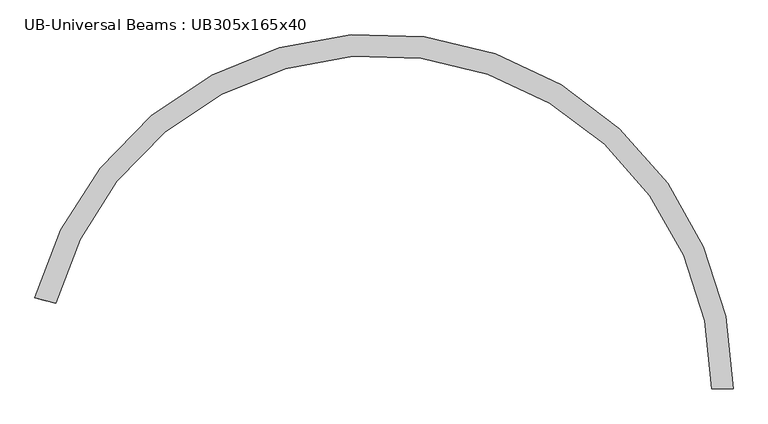
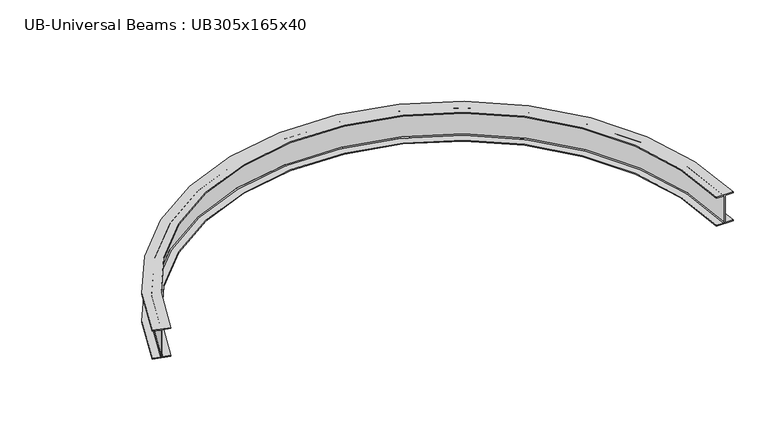
"""IFC4 building model written with IfcOpenShell, lengths in millimetres: beam geometry, UB-Universal Beams : UB305x165x40."""

import ifcopenshell
import ifcopenshell.guid

model = None  # the IFC model being written
_history = None  # IfcOwnerHistory: only IFC2X3 demands one
_inside = {}  # id of a spatial element -> (the spatial element, [elements in it])
_under = {}  # id of a project, library or spatial element -> (it, [spatial elements below it])
_declared = {}  # id of a project -> (the project, [libraries it declares])
_typed = {}  # id of a type object -> (the type object, [elements of that type])
_made_of = {}  # id of a material, layer set ... -> (it, [elements and type objects made of it])


def new_model(schema):
    """Start an empty IFC model of exactly this schema.

    Asked for "IFC4X3", IfcOpenShell would pick the latest addendum, in which some entities
    have other attributes; the version numbers below select the first issue.
    IFC2X3 requires an IfcOwnerHistory on every rooted entity: one is made here for all.
    """
    global model, _history
    if schema == "IFC4X3":
        model = ifcopenshell.file(schema_version=(4, 3, 0, 0))
    else:
        model = ifcopenshell.file(schema=schema)
    _inside.clear()
    _under.clear()
    _declared.clear()
    _typed.clear()
    _made_of.clear()
    _history = None
    if model.schema == "IFC2X3":
        org = make("IfcOrganization", Name="unknown")
        user = make(
            "IfcPersonAndOrganization",
            ThePerson=make("IfcPerson", FamilyName="unknown"),
            TheOrganization=org,
        )
        app = make(
            "IfcApplication",
            ApplicationDeveloper=org,
            Version="unknown",
            ApplicationFullName="unknown",
            ApplicationIdentifier="unknown",
        )
        _history = make(
            "IfcOwnerHistory",
            OwningUser=user,
            OwningApplication=app,
            ChangeAction="ADDED",
            CreationDate=0,
        )
    return model


def make(cls, **values):
    """One entity of the class cls with the attributes given. An attribute that is None is left unset."""
    return model.create_entity(
        cls, **{name: value for name, value in values.items() if value is not None}
    )


def rooted(cls, **values):
    """An entity with a GlobalId (a new one), such as an element, a storey or a relation."""
    return make(cls, GlobalId=ifcopenshell.guid.new(), OwnerHistory=_history, **values)


def si_unit(unit_type, name, prefix=None):
    """IfcSIUnit, for example si_unit("LENGTHUNIT", "METRE", prefix="MILLI")."""
    return make("IfcSIUnit", UnitType=unit_type, Prefix=prefix, Name=name)


def assignment(units):
    """IfcUnitAssignment: the units of a project."""
    return None if units is None else make("IfcUnitAssignment", Units=units)


def point(xyz):
    """IfcCartesianPoint."""
    return None if xyz is None else make("IfcCartesianPoint", Coordinates=xyz)


def direction(xyz):
    """IfcDirection."""
    return None if xyz is None else make("IfcDirection", DirectionRatios=xyz)


def frame(location, z_axis=None, x_axis=None):
    """IfcAxis2Placement3D, a coordinate frame: its origin and axes. An axis left out is left unset."""
    return make(
        "IfcAxis2Placement3D",
        Location=point(location),
        Axis=direction(z_axis),
        RefDirection=direction(x_axis),
    )


def origin():
    """The frame at (0, 0, 0) with its axes left unset."""
    return frame((0.0, 0.0, 0.0))


def place(relative_to, where):
    """IfcLocalPlacement: puts the frame where relative to a parent placement (None: the world)."""
    return make(
        "IfcLocalPlacement", PlacementRelTo=relative_to, RelativePlacement=where
    )


def context(
    kind, dimensions, precision=None, world=None, true_north=None, identifier=None
):
    """IfcGeometricRepresentationContext, for example the 3D "Model" context."""
    return make(
        "IfcGeometricRepresentationContext",
        ContextIdentifier=identifier,
        ContextType=kind,
        CoordinateSpaceDimension=dimensions,
        Precision=precision,
        WorldCoordinateSystem=world,
        TrueNorth=true_north,
    )


def project(units=None, contexts=None):
    """IfcProject with its units and contexts."""
    return rooted(
        "IfcProject",
        Name="project",
        RepresentationContexts=contexts,
        UnitsInContext=assignment(units),
    )


def spatial(cls, under=None, at=None, **own):
    """A site, building, storey or space (cls), placed at a placement, below another one or the project."""
    s = rooted(cls, ObjectPlacement=at, **own)
    if under is not None:
        _under.setdefault(under.id(), (under, []))[1].append(s)
    return s


def polyline(points):
    """IfcPolyline through the points."""
    return make("IfcPolyline", Points=[point(p) for p in points])


def circle_curve(where, radius):
    """IfcCircle in the frame where."""
    return make("IfcCircle", Position=where, Radius=radius)


def ellipse_curve(where, semi_axis1, semi_axis2):
    """IfcEllipse in the frame where."""
    return make(
        "IfcEllipse", Position=where, SemiAxis1=semi_axis1, SemiAxis2=semi_axis2
    )


def trimmed(basis, trim1, trim2, sense, master):
    """IfcTrimmedCurve: the piece of a basis curve between two trims."""
    return make(
        "IfcTrimmedCurve",
        BasisCurve=basis,
        Trim1=trim1,
        Trim2=trim2,
        SenseAgreement=sense,
        MasterRepresentation=master,
    )


def shape(context_of_items, identifier, shape_type, items):
    """IfcShapeRepresentation: the items that make up one representation, for example the "Body"."""
    return make(
        "IfcShapeRepresentation",
        ContextOfItems=context_of_items,
        RepresentationIdentifier=identifier,
        RepresentationType=shape_type,
        Items=items,
    )


def source(mapping_origin, context_of_items, identifier, shape_type, items):
    """IfcRepresentationMap: a shape defined once, which mapped items show again and again."""
    return make(
        "IfcRepresentationMap",
        MappingOrigin=mapping_origin,
        MappedRepresentation=shape(context_of_items, identifier, shape_type, items),
    )


def transform(
    local_origin,
    x_axis=None,
    y_axis=None,
    z_axis=None,
    scale=None,
    scale2=None,
    scale3=None,
    uniform=True,
):
    """IfcCartesianTransformationOperator3D, or its non-uniform kind. x_axis, y_axis, z_axis: its Axis1, 2, 3."""
    if uniform:
        return make(
            "IfcCartesianTransformationOperator3D",
            Axis1=direction(x_axis),
            Axis2=direction(y_axis),
            LocalOrigin=point(local_origin),
            Scale=scale,
            Axis3=direction(z_axis),
        )
    return make(
        "IfcCartesianTransformationOperator3DnonUniform",
        Axis1=direction(x_axis),
        Axis2=direction(y_axis),
        LocalOrigin=point(local_origin),
        Scale=scale,
        Axis3=direction(z_axis),
        Scale2=scale2,
        Scale3=scale3,
    )


def mapped(mapping_source, mapping_target):
    """IfcMappedItem: shows the shape of a source again, moved by a transform."""
    return make(
        "IfcMappedItem", MappingSource=mapping_source, MappingTarget=mapping_target
    )


def made_of(thing, what):
    """Note that an element or type object is made of a material, layer set ...; save() writes the relation."""
    if what is not None:
        _made_of.setdefault(what.id(), (what, []))[1].append(thing)
    return thing


def element(
    cls,
    number,
    at=None,
    inside=None,
    cuts=None,
    type_object=None,
    material=None,
    context=None,
    identifier="Body",
    shape_type=None,
    held_by="IfcProductDefinitionShape",
    body=None,
    shapes=None,
    **own,
):
    """One element of the class cls, such as IfcWall. Its Tag is "e" and its number.

    at: its placement. inside: the storey or other place that contains it. cuts: it is an
    opening in that element (IfcRelVoidsElement). A single representation is given by context,
    identifier, shape_type and body (its items); several are given by shapes. held_by: the class
    of the entity that holds the representations. save() writes the other relations.
    """
    e = rooted(cls, Tag="e%d" % number, ObjectPlacement=at, **own)
    if body is not None:
        shapes = [shape(context, identifier, shape_type, body)]
    if shapes is not None:
        e.Representation = make(held_by, Representations=shapes)
    if inside is not None:
        _inside.setdefault(inside.id(), (inside, []))[1].append(e)
    if cuts is not None:
        rooted(
            "IfcRelVoidsElement", RelatingBuildingElement=cuts, RelatedOpeningElement=e
        )
    if type_object is not None:
        _typed.setdefault(type_object.id(), (type_object, []))[1].append(e)
    return made_of(e, material)


def aggregate(whole, parts):
    """IfcRelAggregates: a whole, such as a stair, and the parts it consists of."""
    return rooted("IfcRelAggregates", RelatingObject=whole, RelatedObjects=parts)


def save(model, path):
    """Write the relations noted so far, then the file.

    IfcRelAggregates (storeys below a building ...), IfcRelContainedInSpatialStructure (elements
    in a storey), IfcRelDefinesByType, IfcRelAssociatesMaterial and IfcRelDeclares: one each for
    every whole, place, type object, material and project.
    """
    for whole, parts in _under.values():
        aggregate(whole, parts)
    for where, things in _inside.values():
        rooted(
            "IfcRelContainedInSpatialStructure",
            RelatedElements=things,
            RelatingStructure=where,
        )
    for kind, things in _typed.values():
        rooted("IfcRelDefinesByType", RelatedObjects=things, RelatingType=kind)
    for what, things in _made_of.values():
        rooted("IfcRelAssociatesMaterial", RelatedObjects=things, RelatingMaterial=what)
    for by, libraries in _declared.values():
        rooted("IfcRelDeclares", RelatingContext=by, RelatedDefinitions=libraries)
    model.write(path)


def plane_surface(at):
    """IfcPlane: the flat surface through the origin of the frame at, square to its z axis."""
    return make("IfcPlane", Position=at)


def cylinder_surface(at, radius):
    """IfcCylindricalSurface: all points at the distance radius from the z axis of the frame at."""
    return make("IfcCylindricalSurface", Position=at, Radius=radius)


def revolved_surface(curve, axis_point, axis_direction):
    """IfcSurfaceOfRevolution: the curve turned about the line through axis_point along axis_direction."""
    return make(
        "IfcSurfaceOfRevolution",
        SweptCurve=make("IfcArbitraryOpenProfileDef", ProfileType="CURVE", Curve=curve),
        AxisPosition=make("IfcAxis1Placement", Location=point(axis_point), Axis=direction(axis_direction)),
    )


def advanced_brep(points, edges, surfaces, faces):
    """IfcAdvancedBrep: a solid bounded by faces that lie on surfaces and meet in shared edges.

    An edge is (start, end): straight between two places in points (the first is 0);
    or (start, end, curve); or (start, end, curve, False) where it runs against its curve.
    A face is (place in surfaces, loops), or (place, loops, False) where it looks against
    its surface's normal. A loop lists edges by number (the first is 1), with a minus sign
    where the edge is run from its end to its start. The first loop is the outer one.
    """
    corners = [point(p) for p in points]
    vertices = [make("IfcVertexPoint", VertexGeometry=c) for c in corners]
    made = []
    for start, end, *more in edges:
        made.append(
            make(
                "IfcEdgeCurve",
                EdgeStart=vertices[start],
                EdgeEnd=vertices[end],
                EdgeGeometry=more[0] if more else make("IfcPolyline", Points=[corners[start], corners[end]]),
                SameSense=more[1] if len(more) > 1 else True,
            )
        )
    hull = []
    for where, loops, *sense in faces:
        bounds = []
        for j, loop in enumerate(loops):
            ring = [make("IfcOrientedEdge", EdgeElement=made[abs(k) - 1], Orientation=k > 0) for k in loop]
            bounds.append(
                make(
                    "IfcFaceOuterBound" if j == 0 else "IfcFaceBound",
                    Bound=make("IfcEdgeLoop", EdgeList=ring),
                    Orientation=True,
                )
            )
        hull.append(make("IfcAdvancedFace", Bounds=bounds, FaceSurface=surfaces[where], SameSense=sense[0] if sense else True))
    return make("IfcAdvancedBrep", Outer=make("IfcClosedShell", CfsFaces=hull))


def ub_universal_beams_ub305x165x40_4e4f8f72(model_context):
    return source(origin(), model_context, "Body", "AdvancedBrep", [
        advanced_brep(
        [(2724.4689627, -2641.9689627, -141.5), (2653.8689627, -2641.9689627, -141.5), (2644.9689627, -2641.9689627, -132.6), (2644.9689627, -2641.9689627, 132.6), (2653.8689627, -2641.9689627, 141.5), (2724.4689627, -2641.9689627, 141.5), (2724.4689627, -2641.9689627, 151.7), (2559.4689627, -2641.9689627, 151.7), (2559.4689627, -2641.9689627, 141.5), (2630.0689627, -2641.9689627, 141.5), (2638.9689627, -2641.9689627, 132.6), (2638.9689627, -2641.9689627, -132.6), (2630.0689627, -2641.9689627, -141.5), (2559.4689627, -2641.9689627, -141.5), (2559.4689627, -2641.9689627, -151.7), (2724.4689627, -2641.9689627, -151.7), (-2633.0924312, -1942.2866222, -141.5), (-2633.0924312, -1942.2866222, -151.7), (-2473.6264005, -1984.6609666, -151.7), (-2473.6264005, -1984.6609666, -141.5), (-2541.8585324, -1966.5298835, -141.5), (-2550.4600335, -1964.244237, -132.6), (-2550.4600335, -1964.244237, 132.6), (-2541.8585324, -1966.5298835, 141.5), (-2473.6264005, -1984.6609666, 141.5), (-2473.6264005, -1984.6609666, 151.7), (-2633.0924312, -1942.2866222, 151.7), (-2633.0924312, -1942.2866222, 141.5), (-2564.8602993, -1960.4177053, 141.5), (-2556.2587982, -1962.7033518, 132.6), (-2556.2587982, -1962.7033518, -132.6), (-2564.8602993, -1960.4177053, -141.5)],
        [
            (0, 1),
            (1, 2, circle_curve(frame((2653.8689627, -2641.9689627, -132.6), z_axis=(0.0, 1.0, 0.0), x_axis=(-1.0, 0.0, 0.0)), 8.9)),
            (2, 3),
            (3, 4, circle_curve(frame((2653.8689627, -2641.9689627, 132.6), z_axis=(0.0, 1.0, 0.0), x_axis=(-1.0, 0.0, 0.0)), 8.9)),
            (4, 5),
            (5, 6),
            (6, 7),
            (7, 8),
            (8, 9),
            (9, 10, circle_curve(frame((2630.0689627, -2641.9689627, 132.6), z_axis=(0.0, 1.0, 0.0), x_axis=(-1.0, 0.0, 0.0)), 8.9)),
            (10, 11),
            (11, 12, circle_curve(frame((2630.0689627, -2641.9689627, -132.6), z_axis=(0.0, 1.0, 0.0), x_axis=(-1.0, 0.0, 0.0)), 8.9)),
            (12, 13),
            (13, 14),
            (14, 15),
            (15, 0),
            (16, 17),
            (17, 18),
            (18, 19),
            (19, 20),
            (20, 21, circle_curve(frame((-2541.8585324, -1966.5298835, -132.6), z_axis=(0.2568142086103926, 0.9664607918875021, 0.0), x_axis=(0.9664607918875021, -0.2568142086103926, 0.0)), 8.9)),
            (21, 22),
            (22, 23, circle_curve(frame((-2541.8585324, -1966.5298835, 132.6), z_axis=(0.2568142086103926, 0.9664607918875021, 0.0), x_axis=(0.9664607918875021, -0.2568142086103926, 0.0)), 8.9)),
            (23, 24),
            (24, 25),
            (25, 26),
            (26, 27),
            (27, 28),
            (28, 29, circle_curve(frame((-2564.8602993, -1960.4177053, 132.6), z_axis=(0.2568142086103926, 0.9664607918875021, 0.0), x_axis=(0.9664607918875021, -0.2568142086103926, 0.0)), 8.9)),
            (29, 30),
            (30, 31, circle_curve(frame((-2564.8602993, -1960.4177053, -132.6), z_axis=(0.2568142086103926, 0.9664607918875021, 0.0), x_axis=(0.9664607918875021, -0.2568142086103926, 0.0)), 8.9)),
            (31, 16),
            (0, 16, circle_curve(frame((0.0, -2641.9689627, -141.5), z_axis=(0.0, 0.0, 1.0), x_axis=(0.0, 1.0, 0.0)), 2724.4689627)),
            (31, 1, circle_curve(frame((0.0, -2641.9689627, -141.5), z_axis=(0.0, 0.0, -1.0), x_axis=(0.0, 1.0, 0.0)), 2653.8689627)),
            (30, 2, circle_curve(frame((0.0, -2641.9689627, -132.6), z_axis=(0.0, 0.0, -1.0), x_axis=(0.0, 1.0, 0.0)), 2644.9689627)),
            (29, 3, circle_curve(frame((0.0, -2641.9689627, 132.6), z_axis=(0.0, 0.0, -1.0), x_axis=(0.0, 1.0, 0.0)), 2644.9689627)),
            (28, 4, circle_curve(frame((0.0, -2641.9689627, 141.5), z_axis=(0.0, 0.0, -1.0), x_axis=(0.0, 1.0, 0.0)), 2653.8689627)),
            (27, 5, circle_curve(frame((0.0, -2641.9689627, 141.5), z_axis=(0.0, 0.0, -1.0), x_axis=(0.0, 1.0, 0.0)), 2724.4689627)),
            (26, 6, circle_curve(frame((0.0, -2641.9689627, 151.7), z_axis=(0.0, 0.0, -1.0), x_axis=(0.0, 1.0, 0.0)), 2724.4689627)),
            (25, 7, circle_curve(frame((0.0, -2641.9689627, 151.7), z_axis=(0.0, 0.0, -1.0), x_axis=(0.0, 1.0, 0.0)), 2559.4689627)),
            (24, 8, circle_curve(frame((0.0, -2641.9689627, 141.5), z_axis=(0.0, 0.0, -1.0), x_axis=(0.0, 1.0, 0.0)), 2559.4689627)),
            (23, 9, circle_curve(frame((0.0, -2641.9689627, 141.5), z_axis=(0.0, 0.0, -1.0), x_axis=(0.0, 1.0, 0.0)), 2630.0689627)),
            (22, 10, circle_curve(frame((0.0, -2641.9689627, 132.6), z_axis=(0.0, 0.0, -1.0), x_axis=(0.0, 1.0, 0.0)), 2638.9689627)),
            (21, 11, circle_curve(frame((0.0, -2641.9689627, -132.6), z_axis=(0.0, 0.0, -1.0), x_axis=(0.0, 1.0, 0.0)), 2638.9689627)),
            (20, 12, circle_curve(frame((0.0, -2641.9689627, -141.5), z_axis=(0.0, 0.0, -1.0), x_axis=(0.0, 1.0, 0.0)), 2630.0689627)),
            (19, 13, circle_curve(frame((0.0, -2641.9689627, -141.5), z_axis=(0.0, 0.0, -1.0), x_axis=(0.0, 1.0, 0.0)), 2559.4689627)),
            (18, 14, circle_curve(frame((0.0, -2641.9689627, -151.7), z_axis=(0.0, 0.0, -1.0), x_axis=(0.0, 1.0, 0.0)), 2559.4689627)),
            (17, 15, circle_curve(frame((0.0, -2641.9689627, -151.7), z_axis=(0.0, 0.0, -1.0), x_axis=(0.0, 1.0, 0.0)), 2724.4689627)),
        ],
        [
            plane_surface(frame((2641.9689627, -2641.9689627, 0.0), z_axis=(0.0, -1.0, 0.0), x_axis=(0.0, 0.0, 1.0))),
            plane_surface(frame((-2553.3594159, -1963.4737944, 0.0), z_axis=(-0.25681420861039306, -0.9664607918875021, 0.0), x_axis=(0.0, 0.0, 1.0))),
            plane_surface(frame((0.0, -2641.9689627, -141.5), z_axis=(0.0, 0.0, 1.0), x_axis=(0.0, 1.0, 0.0))),
            revolved_surface(trimmed(ellipse_curve(frame((0.0, 11.9, -132.6), z_axis=(1.0, 0.0, 0.0), x_axis=(0.0, -1.0, 0.0)), 8.9, 8.9), [point((0.0, 3.0, -132.6))], [point((0.0, 11.9, -141.5))], True, "CARTESIAN"), (0.0, -2641.9689627, 0.0), (0.0, 0.0, -1.0)),
            cylinder_surface(frame((0.0, -2641.9689627, 0.0), z_axis=(0.0, 0.0, -1.0), x_axis=(0.0, 1.0, 0.0)), 2644.9689627),
            revolved_surface(trimmed(ellipse_curve(frame((0.0, 11.9, 132.6), z_axis=(1.0, 0.0, 0.0), x_axis=(0.0, -1.0, 0.0)), 8.9, 8.9), [point((0.0, 11.9, 141.5))], [point((0.0, 3.0, 132.6))], True, "CARTESIAN"), (0.0, -2641.9689627, 0.0), (0.0, 0.0, -1.0)),
            plane_surface(frame((0.0, -2641.9689627, 141.5), z_axis=(0.0, 0.0, -1.0), x_axis=(0.0, 1.0, 0.0))),
            cylinder_surface(frame((0.0, -2641.9689627, 0.0), z_axis=(0.0, 0.0, -1.0), x_axis=(0.0, 1.0, 0.0)), 2724.4689627),
            plane_surface(frame((0.0, -2641.9689627, 151.7), z_axis=(0.0, 0.0, 1.0), x_axis=(0.0, 1.0, 0.0))),
            revolved_surface(polyline([(0.0, -82.5, 141.5), (0.0, -82.5, 151.7)]), (0.0, -2641.9689627, 0.0), (0.0, 0.0, -1.0)),
            revolved_surface(trimmed(ellipse_curve(frame((0.0, -11.9, 132.6), z_axis=(1.0, 0.0, 0.0), x_axis=(0.0, -1.0, 0.0)), 8.9, 8.9), [point((0.0, -3.0, 132.6))], [point((0.0, -11.9, 141.5))], True, "CARTESIAN"), (0.0, -2641.9689627, 0.0), (0.0, 0.0, -1.0)),
            revolved_surface(polyline([(0.0, -3.0, -132.6), (0.0, -3.0, 132.6)]), (0.0, -2641.9689627, 0.0), (0.0, 0.0, -1.0)),
            revolved_surface(trimmed(ellipse_curve(frame((0.0, -11.9, -132.6), z_axis=(1.0, 0.0, 0.0), x_axis=(0.0, -1.0, 0.0)), 8.9, 8.9), [point((0.0, -11.9, -141.5))], [point((0.0, -3.0, -132.6))], True, "CARTESIAN"), (0.0, -2641.9689627, 0.0), (0.0, 0.0, -1.0)),
            revolved_surface(polyline([(0.0, -82.5, -151.7), (0.0, -82.5, -141.5)]), (0.0, -2641.9689627, 0.0), (0.0, 0.0, -1.0)),
            plane_surface(frame((0.0, -2641.9689627, -151.7), z_axis=(0.0, 0.0, -1.0), x_axis=(0.0, 1.0, 0.0))),
        ],
        [
            (0, [[1, 2, 3, 4, 5, 6, 7, 8, 9, 10, 11, 12, 13, 14, 15, 16]]),
            (1, [[17, 18, 19, 20, 21, 22, 23, 24, 25, 26, 27, 28, 29, 30, 31, 32]]),
            (2, [[-1, 33, -32, 34]]),
            (3, [[-2, -34, -31, 35]]),
            (4, [[-3, -35, -30, 36]]),
            (5, [[-4, -36, -29, 37]]),
            (6, [[-5, -37, -28, 38]]),
            (7, [[-6, -38, -27, 39]]),
            (8, [[-7, -39, -26, 40]]),
            (9, [[-8, -40, -25, 41]]),
            (6, [[-9, -41, -24, 42]]),
            (10, [[-10, -42, -23, 43]]),
            (11, [[-11, -43, -22, 44]]),
            (12, [[-12, -44, -21, 45]]),
            (2, [[-13, -45, -20, 46]]),
            (13, [[-14, -46, -19, 47]]),
            (14, [[-15, -47, -18, 48]]),
            (7, [[-16, -48, -17, -33]]),
        ],
    ),
    ])


if __name__ == "__main__":
    model = new_model("IFC4")
    model_context = context("Model", 3, world=origin())
    ifc_project = project(units=[si_unit("LENGTHUNIT", "METRE", prefix="MILLI")], contexts=[model_context])
    site = spatial("IfcSite", under=ifc_project)
    building = spatial("IfcBuilding", under=site)
    placement = place(None, origin())
    ub_universal_beams_ub305x165x40_shape = ub_universal_beams_ub305x165x40_4e4f8f72(model_context)
    element("IfcBeam", 1, ObjectType="UB-Universal Beams : UB305x165x40", at=placement, inside=building, context=model_context, shape_type="MappedRepresentation", body=[
        mapped(ub_universal_beams_ub305x165x40_shape, transform((0.0, 0.0, 0.0), x_axis=(1.0, 0.0, 0.0), y_axis=(0.0, 1.0, 0.0), z_axis=(0.0, 0.0, 1.0))),
    ])
    save(model, "model.ifc")

# Revit data of these elements
# Project information
#   Project Issue Date = "Issue Date"
#   Project Status = "Project Status"
#   Client Name = "Owner"
#   Project Address = "Enter address here"
#   Project Name = "Project Name"
#   Project Number = "0001"
# Type "UB-Universal Beams : UB305x165x40"
#   Section Name Key = "UB305X165X40"
#   Width = 16.5 cm
#   Web Thickness = 0.6 cm
#   Web Fillet = 0.89 cm
#   Warping Constant = 164000.0 cm⁶
#   Torsional Moment of Inertia = 14.70 cm⁴
#   Section Area = 51.3 cm²
#   Plastic Modulus weak axis = 142.0 cm³
#   Plastic Modulus strong axis = 623.0 cm³
#   Nominal Weight = 40.2999 kgf/m
#   Moment of Inertia weak axis = 764.00 cm⁴
#   Moment of Inertia strong axis = 8503.00 cm⁴
#   Height = 30.34 cm
#   Flange Thickness = 1.02 cm
#   Elastic Modulus weak axis = 92.6 cm³
#   Elastic Modulus strong axis = 560.0 cm³
#   Centroid Vertical = 15.17 cm
#   Centroid Horizontal = 8.25 cm
#   Bolt Spacing = 9.0 cm
#   Length [instance default] = 1500 mm
#   Structural Material [instance default] = Metal - Steel 43-275
#   Type Comments = ""
#   Assembly Code = ""
# Element 1 (IfcBeam, "UB-Universal Beams : UB305x165x40")
#   Materials on its faces: "Metal - Steel 43-275"
# Materials
#   "Metal - Steel 43-275": class "Metal", colour RGB 247 247 247, transparency 0, Cost = 0
